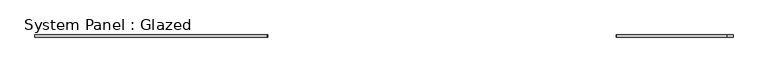
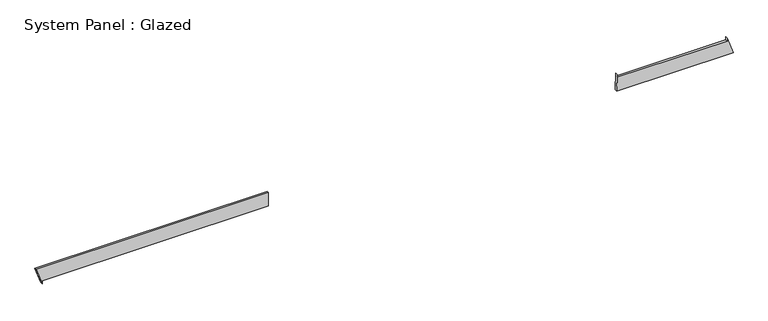
"""IFC4 building model written with IfcOpenShell, lengths in millimetres: plate geometry, System Panel : Glazed."""

from ifc_helpers import new_model, si_unit, frame, origin, place, context, project, spatial, polyline, outline, extrude, source, transform, mapped, element, save


def system_panel_glazed_055f8939(model_context):
    return source(origin(), model_context, "Body", "SweptSolid", [
        extrude(outline(polyline([(35.3553391, 2680.8811306), (35.3553391, 4027.0701191), (235.2094887, 3957.0820623), (199.8541496, 3957.0823635), (199.8433218, 2686.3264609), (235.1986609, 2686.3261596), (35.3553391, 2680.8811306)])), frame((0.0, -49.5, 0.0), z_axis=(0.0, 1.0, 0.0), x_axis=(0.0, 0.0, 1.0)), (0.0, 0.0, 1.0), 25.0),
        extrude(outline(polyline([(0.0, -3956.9205184), (35.3553391, -3956.9205184), (35.3553391, -1342.3654371), (199.8089753, -1344.5935278), (199.7861186, -4027.0701191), (0.0, -3956.9205184)])), frame((0.0, -49.5, 0.0), z_axis=(0.0, 1.0, 0.0), x_axis=(0.0, 0.0, 1.0)), (0.0, 0.0, 1.0), 25.0),
    ])


if __name__ == "__main__":
    model = new_model("IFC4")
    model_context = context("Model", 3, world=origin())
    ifc_project = project(units=[si_unit("LENGTHUNIT", "METRE", prefix="MILLI")], contexts=[model_context])
    site = spatial("IfcSite", under=ifc_project)
    building = spatial("IfcBuilding", under=site)
    placement = place(None, origin())
    system_panel_glazed_shape = system_panel_glazed_055f8939(model_context)
    element("IfcPlate", 1, ObjectType="System Panel : Glazed", at=placement, inside=building, context=model_context, shape_type="MappedRepresentation", body=[
        mapped(system_panel_glazed_shape, transform((0.0, 0.0, 0.0), x_axis=(1.0, 0.0, 0.0), y_axis=(0.0, 1.0, 0.0), z_axis=(0.0, 0.0, 1.0))),
    ])
    save(model, "model.ifc")

# Revit data of these elements
# Element 1 (IfcPlate, "System Panel : Glazed")
#   Materials on its faces: "Glass"
# Materials
#   "Glass": class "Glass", colour RGB 218 227 224, transparency 0.85, Description = "Soda Lime Glass", Cost = 0
